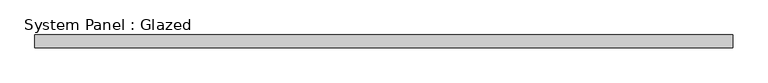
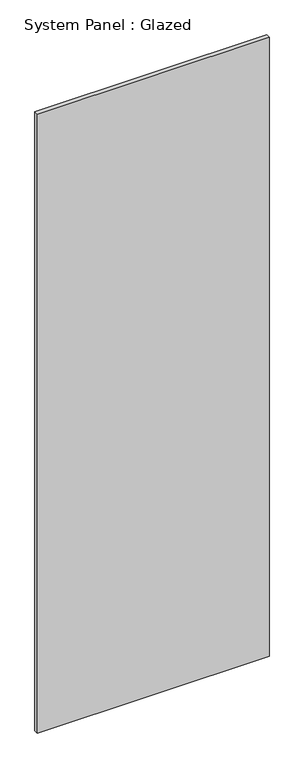
"""IFC4 building model written with IfcOpenShell, lengths in millimetres: plate geometry, System Panel : Glazed."""

from ifc_helpers import new_model, si_unit, origin, origin_with_axes, place, context, project, spatial, polyline, outline, extrude, source, transform, mapped, element, save


def system_panel_glazed_78b5b18d(model_context):
    return source(origin(), model_context, "Body", "SweptSolid", [
        extrude(outline(polyline([(691.7836538, 19.05), (-691.7836538, 19.05), (-691.7836538, 44.45), (691.7836538, 44.45), (691.7836538, 19.05)])), origin_with_axes(), (0.0, 0.0, 1.0), 3908.2835741),
    ])


if __name__ == "__main__":
    model = new_model("IFC4")
    model_context = context("Model", 3, world=origin())
    ifc_project = project(units=[si_unit("LENGTHUNIT", "METRE", prefix="MILLI")], contexts=[model_context])
    site = spatial("IfcSite", under=ifc_project)
    building = spatial("IfcBuilding", under=site)
    placement = place(None, origin())
    system_panel_glazed_shape = system_panel_glazed_78b5b18d(model_context)
    element("IfcPlate", 1, ObjectType="System Panel : Glazed", at=placement, inside=building, context=model_context, shape_type="MappedRepresentation", body=[
        mapped(system_panel_glazed_shape, transform((0.0, 0.0, 0.0), x_axis=(1.0, 0.0, 0.0), y_axis=(0.0, 1.0, 0.0), z_axis=(0.0, 0.0, 1.0))),
    ])
    save(model, "model.ifc")

# Revit data of these elements
# Type "System Panel : Glazed"
#   Construction Type Id = "GSP4R"
#   Analytic Construction = "1/8 in Pilkington single glazing"
#   Visual Light Transmittance = 0.9
#   Solar Heat Gain Coefficient = 0.86
#   Heat Transfer Coefficient (U) = 1.18115 BTU/(h·ft²·°F)
#   Define Thermal Properties by = 1
# Element 1 (IfcPlate, "System Panel : Glazed")
#   Materials on its faces: "Glass"
# Materials
#   "Glass": class "Glass", colour RGB 0 128 192, transparency 0.75, Description = "Soda Lime Glass", Cost = 0
